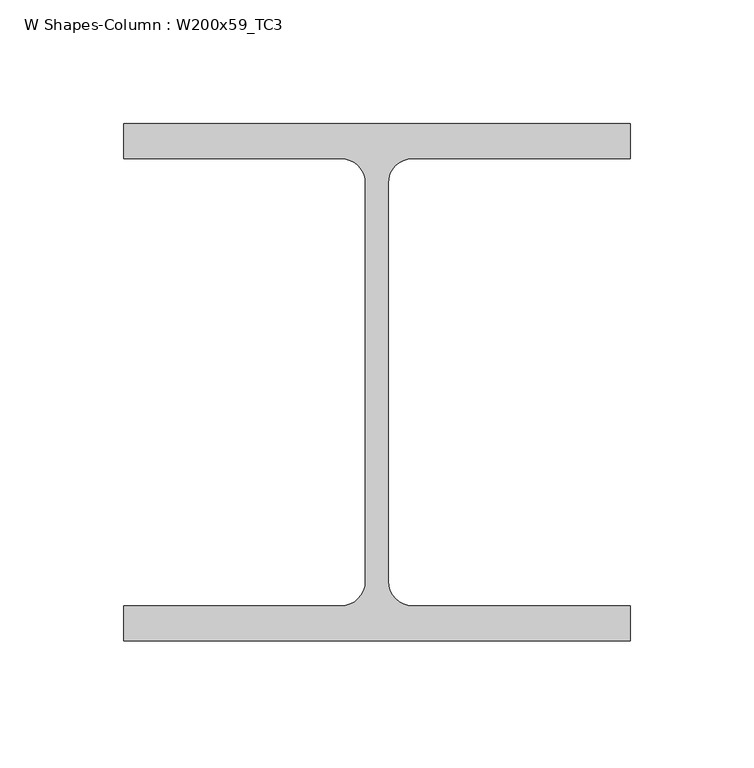
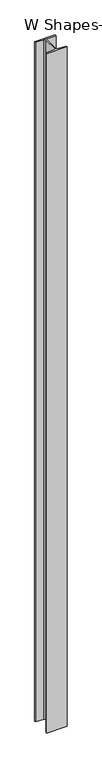
"""IFC4 building model written with IfcOpenShell, lengths in millimetres: column geometry, W Shapes-Column : W200x59_TC3."""

from ifc_helpers import new_model, si_unit, point, frame, frame_2d, origin, place, context, project, spatial, polyline, circle_curve, trimmed, segment, composite_curve, outline, extrude, source, transform, mapped, element, save


def w_shapes_column_w200x59_tc3_ad9554a8(model_context):
    return source(origin(), model_context, "Body", "SweptSolid", [
        extrude(outline(composite_curve([segment(polyline([(102.489, 104.775), (102.489, 90.551), (14.5796, 90.551)]), True, "CONTINUOUS"), segment(trimmed(circle_curve(frame_2d((14.5796, 80.5434)), 10.0076), [point((14.5796, 90.551))], [point((4.572, 80.5434))], True, "CARTESIAN"), True, "CONTINUOUS"), segment(polyline([(4.572, 80.5434), (4.572, -80.5434)]), True, "CONTINUOUS"), segment(trimmed(circle_curve(frame_2d((14.5796, -80.5434)), 10.0076), [point((4.572, -80.5434))], [point((14.5796, -90.551))], True, "CARTESIAN"), True, "CONTINUOUS"), segment(polyline([(14.5796, -90.551), (102.489, -90.551), (102.489, -104.775), (-102.489, -104.775), (-102.489, -90.551), (-14.5796, -90.551)]), True, "CONTINUOUS"), segment(trimmed(circle_curve(frame_2d((-14.5796, -80.5434)), 10.0076), [point((-14.5796, -90.551))], [point((-4.572, -80.5434))], True, "CARTESIAN"), True, "CONTINUOUS"), segment(polyline([(-4.572, -80.5434), (-4.572, 80.5434)]), True, "CONTINUOUS"), segment(trimmed(circle_curve(frame_2d((-14.5796, 80.5434)), 10.0076), [point((-4.572, 80.5434))], [point((-14.5796, 90.551))], True, "CARTESIAN"), True, "CONTINUOUS"), segment(polyline([(-14.5796, 90.551), (-102.489, 90.551), (-102.489, 104.775), (102.489, 104.775)]), True, "CONTINUOUS")], self_intersect=False)), frame((0.0, 0.0, 200.0), z_axis=(0.0, 0.0, 1.0), x_axis=(1.0, 0.0, 0.0)), (0.0, 0.0, 1.0), 7250.0),
    ])


if __name__ == "__main__":
    model = new_model("IFC4")
    model_context = context("Model", 3, world=origin())
    ifc_project = project(units=[si_unit("LENGTHUNIT", "METRE", prefix="MILLI")], contexts=[model_context])
    site = spatial("IfcSite", under=ifc_project)
    building = spatial("IfcBuilding", under=site)
    placement = place(None, origin())
    w_shapes_column_w200x59_tc3_shape = w_shapes_column_w200x59_tc3_ad9554a8(model_context)
    element("IfcColumn", 1, ObjectType="W Shapes-Column : W200x59_TC3", at=placement, inside=building, context=model_context, shape_type="MappedRepresentation", body=[
        mapped(w_shapes_column_w200x59_tc3_shape, transform((0.0, 0.0, 0.0), x_axis=(1.0, 0.0, 0.0), y_axis=(0.0, 1.0, 0.0), z_axis=(0.0, 0.0, 1.0))),
    ])
    save(model, "model.ifc")

# Revit data of these elements
# Type "W Shapes-Column : W200x59_TC3"
#   Section Name Key = "W8X40"
#   Assembly Code = "B10"
#   Width = 20.4978 cm
#   Web Thickness = 0.9144 cm
#   Web Fillet = 1.0008 cm
#   Warping Constant = 194957.0 cm⁶
#   Torsional Moment of Inertia = 46.6179 cm⁴
#   Section Area = 75.4837 cm²
#   Plastic Modulus weak axis = 303.161 cm³
#   Plastic Modulus strong axis = 652.205 cm³
#   Perimeter = 1.20396 m²/m
#   Nominal Weight = 59.5266 kgf/m
#   Moment of Inertia weak axis = 2043.70 cm⁴
#   Moment of Inertia strong axis = 6076.98 cm⁴
#   Height = 20.955 cm
#   Flange Thickness = 1.4224 cm
#   Elastic Modulus weak axis = 199.922 cm³
#   Elastic Modulus strong axis = 581.741 cm³
#   Clear Web Height = 14.605 cm
#   Centroid Vertical = 10.4775 cm
#   Centroid Horizontal = 10.2489 cm
#   Bolt Spacing = 13.97 cm
#   Structural Material [instance default] = Steel ASTM A992
#   Principal Axes Angle = 0
# Element 1 (IfcColumn, "W Shapes-Column : W200x59_TC3")
#   Structural Material = none
# Materials
#   "Steel ASTM A992": class "Metal", colour RGB 199 199 199, transparency 0, Description = "Structural steel 50ksi", Cost = 0
